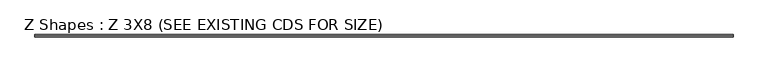
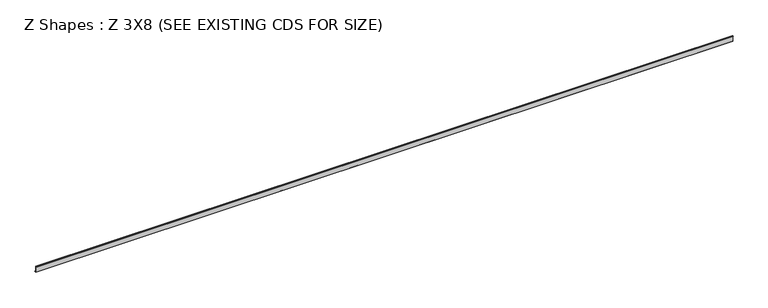
"""IFC4 building model written with IfcOpenShell, lengths in millimetres: beam geometry, Z Shapes : Z 3X8 (SEE EXISTING CDS FOR SIZE)."""

from ifc_helpers import new_model, si_unit, frame, origin, place, context, project, spatial, polyline, outline, extrude, source, transform, mapped, element, save


def z_shapes_z_3x8_see_existing_cds_for_size_e2318bef(model_context):
    return source(origin(), model_context, "Body", "SweptSolid", [
        extrude(outline(polyline([(-57.2805719, 91.944825), (-57.2805719, 101.596825), (-19.1805719, 101.596825), (-19.1805719, -91.951175), (18.9194281, -91.951175), (18.9194281, -101.603175), (-25.0225719, -101.603175), (-25.0225719, 91.944825), (-57.2805719, 91.944825)])), frame((-11671.3, 0.0, 0.0), z_axis=(1.0, 0.0, 0.0), x_axis=(0.0, 1.0, 0.0)), (0.0, 0.0, 1.0), 23342.6),
    ])


if __name__ == "__main__":
    model = new_model("IFC4")
    model_context = context("Model", 3, world=origin())
    ifc_project = project(units=[si_unit("LENGTHUNIT", "METRE", prefix="MILLI")], contexts=[model_context])
    site = spatial("IfcSite", under=ifc_project)
    building = spatial("IfcBuilding", under=site)
    placement = place(None, origin())
    z_shapes_z_3x8_see_existing_cds_for_size_shape = z_shapes_z_3x8_see_existing_cds_for_size_e2318bef(model_context)
    element("IfcBeam", 1, ObjectType="Z Shapes : Z 3X8 (SEE EXISTING CDS FOR SIZE)", at=placement, inside=building, context=model_context, shape_type="MappedRepresentation", body=[
        mapped(z_shapes_z_3x8_see_existing_cds_for_size_shape, transform((0.0, 0.0, 0.0), x_axis=(1.0, 0.0, 0.0), y_axis=(0.0, 1.0, 0.0), z_axis=(0.0, 0.0, 1.0))),
    ])
    save(model, "model.ifc")

# Revit data of these elements
# Type "Z Shapes : Z 3X8 (SEE EXISTING CDS FOR SIZE)"
#   Section Name Key = "W12x26"
#   Assembly Code = "B10"
#   Width = 76.2 mm
#   Web Thickness = 5.842 mm
#   Web Fillet = 7.62 mm
#   Warping Constant = 163001.3 cm⁶
#   Torsional Moment of Inertia = 12.4869 cm⁴
#   Section Area = 7.65 in²
#   Plastic Modulus weak axis = 0.00472801 (stored number, unit not read)
#   Plastic Modulus strong axis = 0.0215278 (stored number, unit not read)
#   Perimeter = 15.0571 m²/m
#   Nominal Weight = 379.441 N/m
#   Moment of Inertia weak axis = 720.08 cm⁴
#   Moment of Inertia strong axis = 8491.12 cm⁴
#   Height = 203.2 mm
#   Flange Thickness = 9.652 mm
#   Elastic Modulus weak axis = 0.00309028 (stored number, unit not read)
#   Elastic Modulus strong axis = 0.0193287 (stored number, unit not read)
#   Centroid Vertical = 101.6 mm
#   Centroid Horizontal = 38.1 mm
#   Length [instance default] = 5' - 0"
#   Structural Material [instance default] = Steel ASTM A992
#   Principal Axes Angle = 0
# Element 1 (IfcBeam, "Z Shapes : Z 3X8 (SEE EXISTING CDS FOR SIZE)")
#   Structural Material = PAINTED STEEL
#   Materials on its faces: "PAINTED STEEL"
# Materials
#   "Steel ASTM A992": class "Metal", colour RGB 189 187 185, transparency 0, Description = "Structural steel 50ksi", Cost = 0
#   "PAINTED STEEL": class "Generic", colour RGB 120 120 120, transparency 0, Cost = 0
